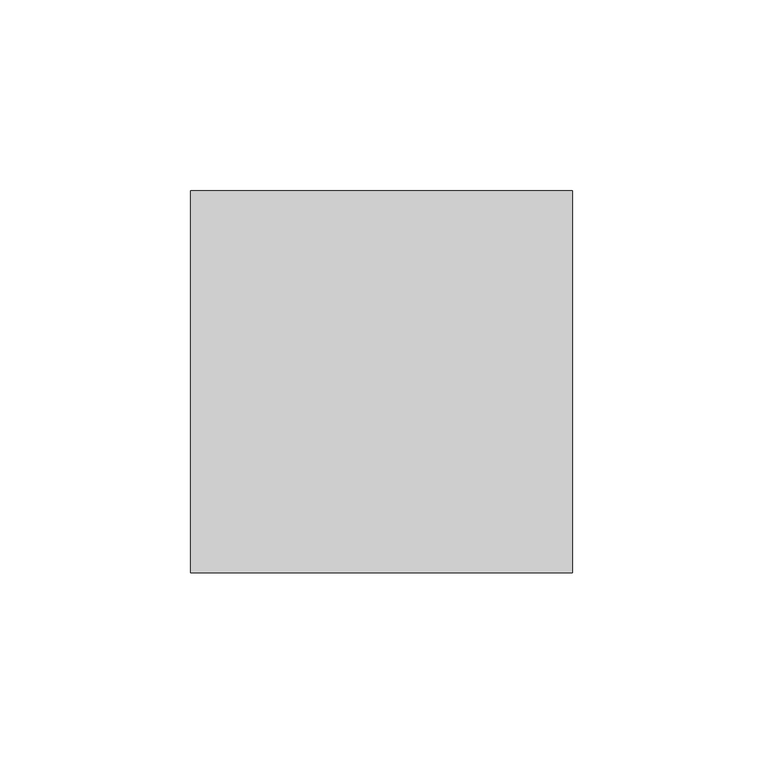
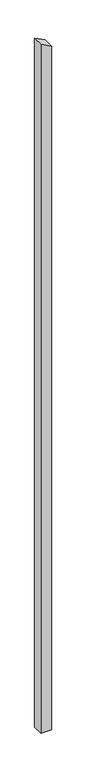
"""IFC4 building model written with IfcOpenShell, lengths in millimetres: column geometry, Holzstütze 159056 : Holzstütze 159056."""

from ifc_helpers import new_model, si_unit, frame, origin, place, context, project, spatial, polyline, outline, extrude, source, transform, mapped, element, save


def column_ed14f447(model_context):
    return source(origin(), model_context, "Body", "SweptSolid", [
        extrude(outline(polyline([(-500.0, 174197.7593015), (-500.0, 174297.7593015), (6345.7118258, 174297.7593015), (6396.6643707, 174197.7593015), (-500.0, 174197.7593015)])), frame((0.0, 29551.5369795, 0.0), z_axis=(0.0, 1.0, 0.0), x_axis=(0.0, 0.0, 1.0)), (0.0, 0.0, 1.0), 100.0),
    ])


if __name__ == "__main__":
    model = new_model("IFC4")
    model_context = context("Model", 3, world=origin())
    ifc_project = project(units=[si_unit("LENGTHUNIT", "METRE", prefix="MILLI")], contexts=[model_context])
    site = spatial("IfcSite", under=ifc_project)
    building = spatial("IfcBuilding", under=site)
    placement = place(None, origin())
    column_shape = column_ed14f447(model_context)
    element("IfcColumn", 1, ObjectType="Holzstütze 159056 : Holzstütze 159056", at=placement, inside=building, context=model_context, shape_type="MappedRepresentation", body=[
        mapped(column_shape, transform((0.0, 0.0, 0.0), x_axis=(1.0, 0.0, 0.0), y_axis=(0.0, 1.0, 0.0), z_axis=(0.0, 0.0, 1.0))),
    ])
    save(model, "model.ifc")

# Revit data of these elements
# Type "Holzstütze 159056 : Holzstütze 159056"
#   Abrechnungsart = "m"
#   Allright_Bauteil_ID = "0152St 0000143490"
#   Bezeichnung = "Holzstütze"
#   Codetext = "ST-HOLZ\\"
#   Gewerk = "Zimmer- und Holzbauarbeiten"
#   Material = "Holz"
#   Objektname = "Stütze"
#   NameOverride = "Holzstütze"
#   Reference = "Holzstütze"
#   Status = "NEW"
#   ThermalTransmittance = 0.0000 BTU/(h·ft²·°F)
#   Roll = 0.00°
#   Slope = 0.00°
#   2D Interaktion = yes
#   IsExternal = yes
#   LoadBearing = yes
# Element 1 (IfcColumn, "Holzstütze 159056 : Holzstütze 159056")
#   Materials on its faces: "holzschalung"
# Materials
#   "holzschalung": class "Unassigned", colour RGB 128 128 128, transparency 0
